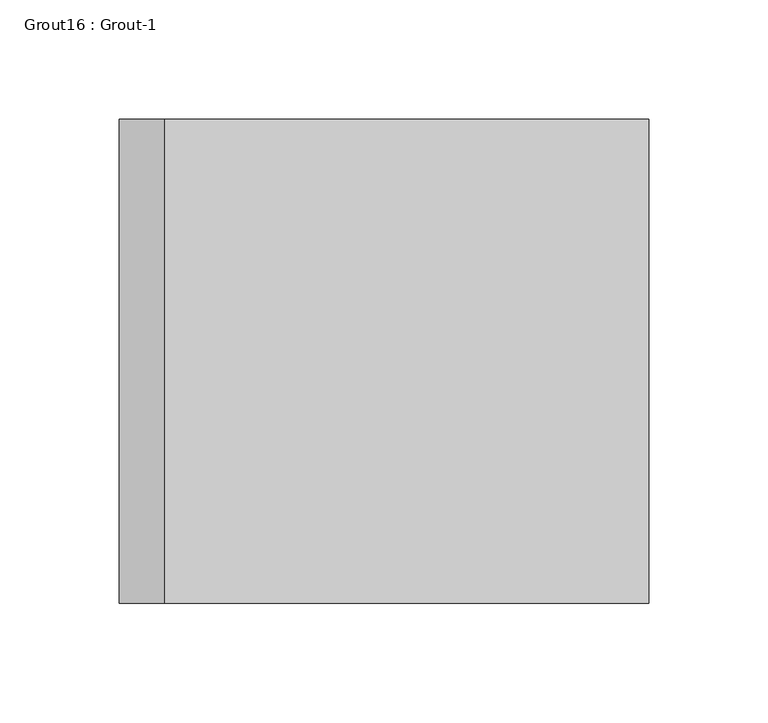
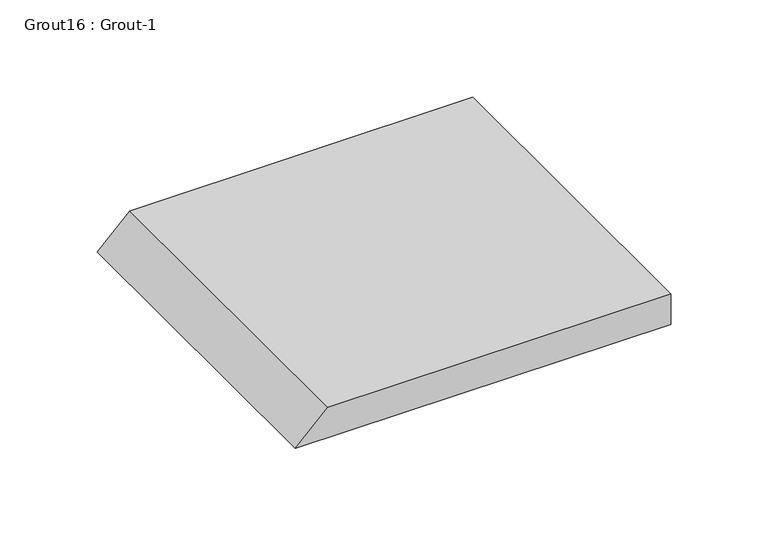
"""IFC4 building model written with IfcOpenShell, lengths in millimetres: proxy geometry, Grout16 : Grout-1."""

from ifc_helpers import new_model, si_unit, frame, origin, place, context, project, spatial, polyline, outline, extrude, source, transform, mapped, element, save


def grout16_grout_1_e9fd96e3(model_context):
    return source(origin(), model_context, "Body", "SweptSolid", [
        extrude(outline(polyline([(19.05, 590115.4434739), (0.0, 590096.3934739), (0.0, 590318.6434739), (19.05, 590318.6434739), (19.05, 590115.4434739)])), frame((0.0, -534144.2913841, 0.0), z_axis=(0.0, 1.0, 0.0), x_axis=(0.0, 0.0, 1.0)), (0.0, 0.0, 1.0), 203.2),
    ])


if __name__ == "__main__":
    model = new_model("IFC4")
    model_context = context("Model", 3, world=origin())
    ifc_project = project(units=[si_unit("LENGTHUNIT", "METRE", prefix="MILLI")], contexts=[model_context])
    site = spatial("IfcSite", under=ifc_project)
    building = spatial("IfcBuilding", under=site)
    placement = place(None, origin())
    grout16_grout_1_shape = grout16_grout_1_e9fd96e3(model_context)
    element("IfcBuildingElementProxy", 1, Name="Grout16 : Grout-1", ObjectType="Grout16 : Grout-1", at=placement, inside=building, context=model_context, shape_type="MappedRepresentation", body=[
        mapped(grout16_grout_1_shape, transform((0.0, 0.0, 0.0), x_axis=(1.0, 0.0, 0.0), y_axis=(0.0, 1.0, 0.0), z_axis=(0.0, 0.0, 1.0))),
    ])
    save(model, "model.ifc")

# Revit data of these elements
# Element 1 (IfcBuildingElementProxy, "Grout16 : Grout-1")
#   Materials on its faces: "3/4\" NON SHRINK GROUT"
# Materials
#   "3/4\" NON SHRINK GROUT": class "Generic", colour RGB 145 145 143, transparency 0, Cost = 0
